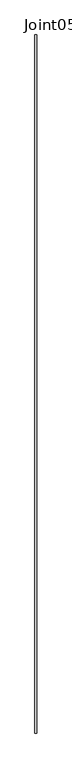
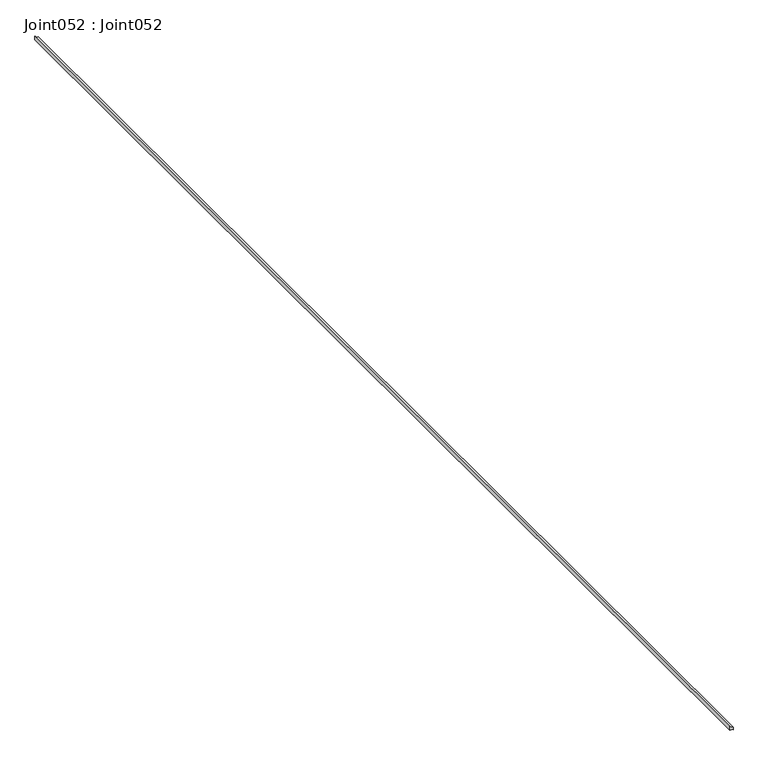
"""IFC4 building model written with IfcOpenShell, lengths in millimetres: proxy geometry, Joint052 : Joint052."""

from ifc_helpers import new_model, si_unit, point, frame, frame_2d, origin, place, context, project, spatial, polyline, circle_curve, trimmed, segment, composite_curve, outline, extrude, source, transform, mapped, element, save


def joint052_joint052_3b431e29(model_context):
    return source(origin(), model_context, "Body", "SweptSolid", [
        extrude(outline(composite_curve([segment(trimmed(circle_curve(frame_2d((42762.4796982, 6173.4695181)), 6.2056875), [point((42768.3524673, 6171.4642399))], [point((42767.5722366, 6177.0158698))], True, "CARTESIAN"), True, "CONTINUOUS"), segment(polyline([(42767.5722366, 6177.0158698), (42771.7794904, 6177.0158698)]), True, "CONTINUOUS"), segment(trimmed(circle_curve(frame_2d((42777.555878, 6176.765693)), 5.7818027), [point((42771.7794904, 6177.0158698))], [point((42775.2485338, 6171.4642399))], True, "CARTESIAN"), True, "CONTINUOUS"), segment(polyline([(42775.2485338, 6171.4642399), (42768.3524673, 6171.4642399)]), True, "CONTINUOUS")], self_intersect=False)), frame((0.0, -1052.891, 0.0), z_axis=(0.0, 1.0, 0.0), x_axis=(0.0, 0.0, 1.0)), (0.0, 0.0, 1.0), 2000.0),
    ])


if __name__ == "__main__":
    model = new_model("IFC4")
    model_context = context("Model", 3, world=origin())
    ifc_project = project(units=[si_unit("LENGTHUNIT", "METRE", prefix="MILLI")], contexts=[model_context])
    site = spatial("IfcSite", under=ifc_project)
    building = spatial("IfcBuilding", under=site)
    placement = place(None, origin())
    joint052_joint052_shape = joint052_joint052_3b431e29(model_context)
    element("IfcBuildingElementProxy", 1, Name="Joint052 : Joint052", ObjectType="Joint052 : Joint052", at=placement, inside=building, context=model_context, shape_type="MappedRepresentation", body=[
        mapped(joint052_joint052_shape, transform((0.0, 0.0, 0.0), x_axis=(1.0, 0.0, 0.0), y_axis=(0.0, 1.0, 0.0), z_axis=(0.0, 0.0, 1.0))),
    ])
    save(model, "model.ifc")

# Revit data of these elements
# Type "Joint052 : Joint052"
#   NameOverride = "Joint052"
# Element 1 (IfcBuildingElementProxy, "Joint052 : Joint052")
#   Materials on its faces: "SEALANT"
# Materials
#   "SEALANT": class "Unassigned", colour RGB 142 225 148, transparency 0
